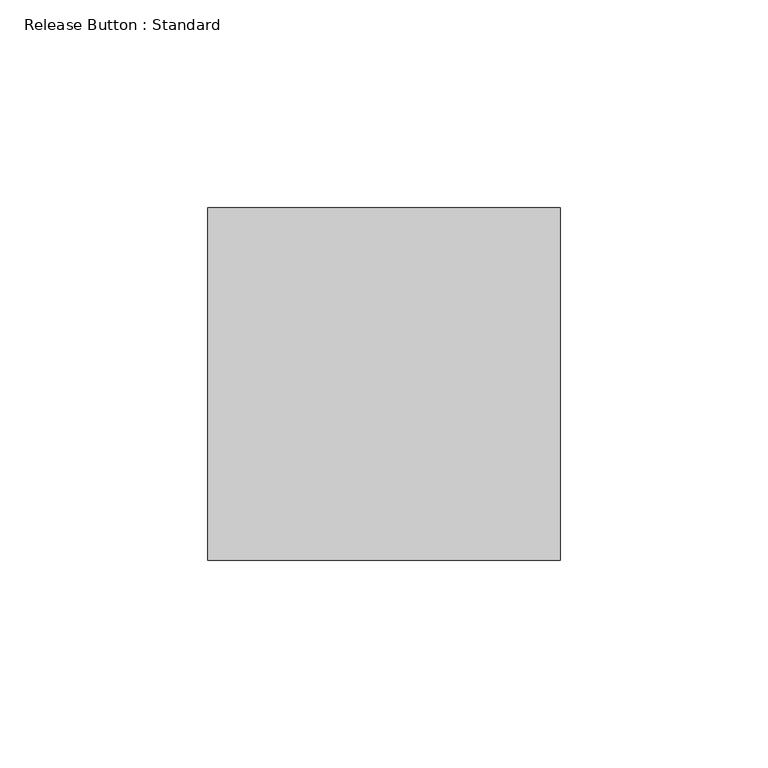
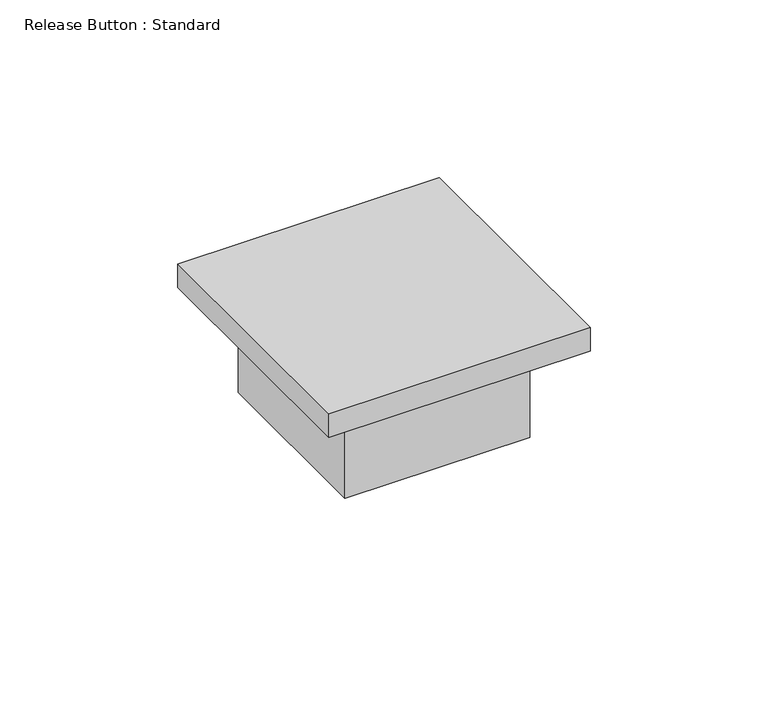
"""IFC4 building model written with IfcOpenShell, lengths in millimetres: proxy geometry, Release Button : Standard."""

from ifc_helpers import new_model, si_unit, frame, origin, origin_with_axes, place, context, project, spatial, polyline, outline, extrude, source, transform, mapped, element, save


def release_button_standard_0a205331(model_context):
    return source(origin(), model_context, "Body", "SweptSolid", [
        extrude(outline(polyline([(42.5, -85.0), (-42.5, -85.0), (-42.5, 0.0), (42.5, 0.0), (42.5, -85.0)])), origin_with_axes(), (0.0, 0.0, 1.0), 8.0),
        extrude(outline(polyline([(30.0, -72.5), (-30.0, -72.5), (-30.0, -12.5), (30.0, -12.5), (30.0, -72.5)])), frame((0.0, 0.0, -33.0), z_axis=(0.0, 0.0, 1.0), x_axis=(1.0, 0.0, 0.0)), (0.0, 0.0, 1.0), 33.0),
    ])


if __name__ == "__main__":
    model = new_model("IFC4")
    model_context = context("Model", 3, world=origin())
    ifc_project = project(units=[si_unit("LENGTHUNIT", "METRE", prefix="MILLI")], contexts=[model_context])
    site = spatial("IfcSite", under=ifc_project)
    building = spatial("IfcBuilding", under=site)
    placement = place(None, origin())
    release_button_standard_shape = release_button_standard_0a205331(model_context)
    element("IfcBuildingElementProxy", 1, Name="Release Button : Standard", ObjectType="Release Button : Standard", at=placement, inside=building, context=model_context, shape_type="MappedRepresentation", body=[
        mapped(release_button_standard_shape, transform((0.0, 0.0, 0.0), x_axis=(1.0, 0.0, 0.0), y_axis=(0.0, 1.0, 0.0), z_axis=(0.0, 0.0, 1.0))),
    ])
    save(model, "model.ifc")

# Revit data of these elements
# Type "Release Button : Standard"
#   Type Mark = "Release Button"
#   Classification.OmniClass.21.Number = "21-04 70 10 10"
#   Classification.OmniClass.21.Description = "Access Control"
#   Classification.OmniClass.23.Number = "23-29 13 00"
#   Classification.OmniClass.23.Description = "Security Access Controls"
#   COBie.Type.CreatedBy = "info@mma.ie"
#   COBie.Type.CreatedOn = "2017-07-26T09:12:44"
#   COBie.Type.Name = "Release Button"
#   COBie.Type.Category = "23-29 13 00 : Security Access Controls"
#   COBie.Type.Description = "Release Button_Standard"
#   COBie.Type.AssetType = "Fixed"
#   COBie.Type.Manufacturer = ""
#   COBie.Type.ModelNumber = ""
#   COBie.Type.ModelReference = ""
#   COBie.Type.Color = "Stainless Steel"
#   Units = "Volts"
#   Keynote = "28 13 00.C"
#   COBie.Type.ReplacementCost = 0
#   RB_Width = 85 mm
#   RB_Height = 85 mm
#   RB_Depth = 41 mm
#   Default Elevation = 1200 mm
#   COBie.Type = yes
#   URL = ""
#   Model = ""
#   Manufacturer = ""
